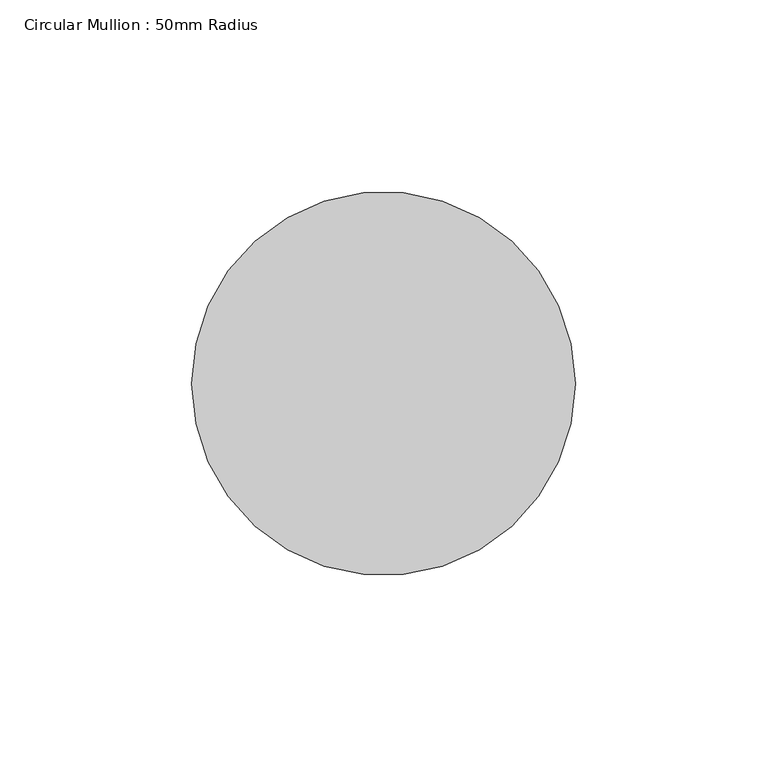
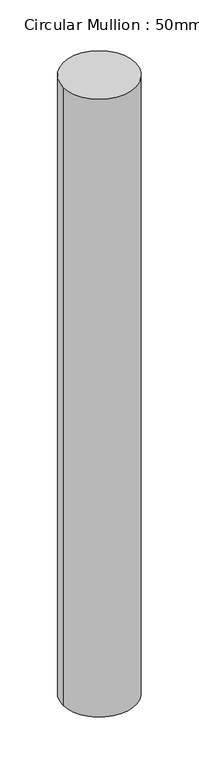
"""IFC4 building model written with IfcOpenShell, lengths in millimetres: member geometry, Circular Mullion : 50mm Radius."""

from ifc_helpers import new_model, si_unit, point, frame, origin, origin_2d, place, context, project, spatial, circle_curve, trimmed, segment, composite_curve, outline, extrude, source, transform, mapped, element, save


def circular_mullion_50mm_radius_e1fb1ca7(model_context):
    return source(origin(), model_context, "Body", "SweptSolid", [
        extrude(outline(composite_curve([segment(trimmed(circle_curve(origin_2d(), 50.0), [point((50.0, 0.0))], [point((-50.0, 0.0))], False, "CARTESIAN"), True, "CONTINUOUS"), segment(trimmed(circle_curve(origin_2d(), 50.0), [point((-50.0, 0.0))], [point((50.0, 0.0))], False, "CARTESIAN"), True, "CONTINUOUS")], self_intersect=False)), frame((0.0, 0.0, -896.8634355), z_axis=(0.0, 0.0, 1.0), x_axis=(1.0, 0.0, 0.0)), (0.0, 0.0, 1.0), 896.8634355),
    ])


if __name__ == "__main__":
    model = new_model("IFC4")
    model_context = context("Model", 3, world=origin())
    ifc_project = project(units=[si_unit("LENGTHUNIT", "METRE", prefix="MILLI")], contexts=[model_context])
    site = spatial("IfcSite", under=ifc_project)
    building = spatial("IfcBuilding", under=site)
    placement = place(None, origin())
    circular_mullion_50mm_radius_shape = circular_mullion_50mm_radius_e1fb1ca7(model_context)
    element("IfcMember", 1, ObjectType="Circular Mullion : 50mm Radius", at=placement, inside=building, context=model_context, shape_type="MappedRepresentation", body=[
        mapped(circular_mullion_50mm_radius_shape, transform((0.0, 0.0, 0.0), x_axis=(1.0, 0.0, 0.0), y_axis=(0.0, 1.0, 0.0), z_axis=(0.0, 0.0, 1.0))),
    ])
    save(model, "model.ifc")

# Revit data of these elements
# Type "Circular Mullion : 50mm Radius"
#   built-in parameter 1007350 = 0.164042 (stored number, unit not read)
# Element 1 (IfcMember, "Circular Mullion : 50mm Radius")
#   Materials on its faces: "Aluminium"
# Materials
#   "Aluminium": class "Metal", colour RGB 247 247 247, transparency 0, Description = "Aluminium 6061", Cost = 0
